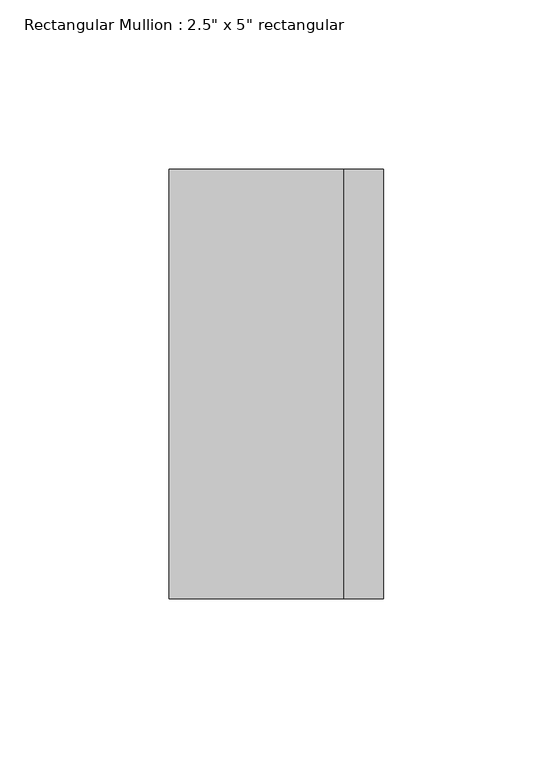
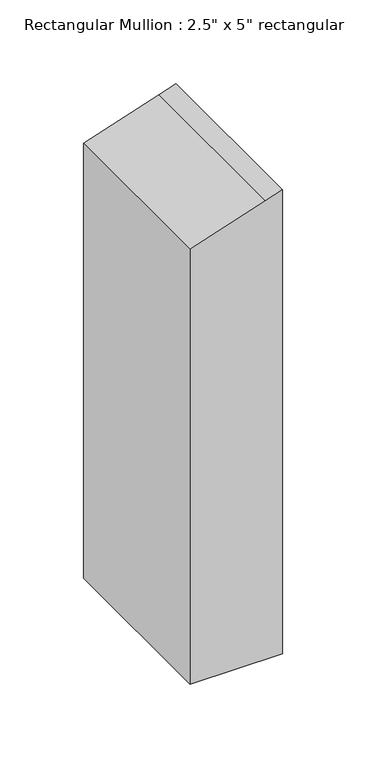
"""IFC4 building model written with IfcOpenShell, lengths in millimetres: member geometry."""

import ifcopenshell
import ifcopenshell.guid

model = None  # the IFC model being written
_history = None  # IfcOwnerHistory: only IFC2X3 demands one
_inside = {}  # id of a spatial element -> (the spatial element, [elements in it])
_under = {}  # id of a project, library or spatial element -> (it, [spatial elements below it])
_declared = {}  # id of a project -> (the project, [libraries it declares])
_typed = {}  # id of a type object -> (the type object, [elements of that type])
_made_of = {}  # id of a material, layer set ... -> (it, [elements and type objects made of it])


def new_model(schema):
    """Start an empty IFC model of exactly this schema.

    Asked for "IFC4X3", IfcOpenShell would pick the latest addendum, in which some entities
    have other attributes; the version numbers below select the first issue.
    IFC2X3 requires an IfcOwnerHistory on every rooted entity: one is made here for all.
    """
    global model, _history
    if schema == "IFC4X3":
        model = ifcopenshell.file(schema_version=(4, 3, 0, 0))
    else:
        model = ifcopenshell.file(schema=schema)
    _inside.clear()
    _under.clear()
    _declared.clear()
    _typed.clear()
    _made_of.clear()
    _history = None
    if model.schema == "IFC2X3":
        org = make("IfcOrganization", Name="unknown")
        user = make(
            "IfcPersonAndOrganization",
            ThePerson=make("IfcPerson", FamilyName="unknown"),
            TheOrganization=org,
        )
        app = make(
            "IfcApplication",
            ApplicationDeveloper=org,
            Version="unknown",
            ApplicationFullName="unknown",
            ApplicationIdentifier="unknown",
        )
        _history = make(
            "IfcOwnerHistory",
            OwningUser=user,
            OwningApplication=app,
            ChangeAction="ADDED",
            CreationDate=0,
        )
    return model


def make(cls, **values):
    """One entity of the class cls with the attributes given. An attribute that is None is left unset."""
    return model.create_entity(
        cls, **{name: value for name, value in values.items() if value is not None}
    )


def rooted(cls, **values):
    """An entity with a GlobalId (a new one), such as an element, a storey or a relation."""
    return make(cls, GlobalId=ifcopenshell.guid.new(), OwnerHistory=_history, **values)


def si_unit(unit_type, name, prefix=None):
    """IfcSIUnit, for example si_unit("LENGTHUNIT", "METRE", prefix="MILLI")."""
    return make("IfcSIUnit", UnitType=unit_type, Prefix=prefix, Name=name)


def assignment(units):
    """IfcUnitAssignment: the units of a project."""
    return None if units is None else make("IfcUnitAssignment", Units=units)


def point(xyz):
    """IfcCartesianPoint."""
    return None if xyz is None else make("IfcCartesianPoint", Coordinates=xyz)


def direction(xyz):
    """IfcDirection."""
    return None if xyz is None else make("IfcDirection", DirectionRatios=xyz)


def frame(location, z_axis=None, x_axis=None):
    """IfcAxis2Placement3D, a coordinate frame: its origin and axes. An axis left out is left unset."""
    return make(
        "IfcAxis2Placement3D",
        Location=point(location),
        Axis=direction(z_axis),
        RefDirection=direction(x_axis),
    )


def origin():
    """The frame at (0, 0, 0) with its axes left unset."""
    return frame((0.0, 0.0, 0.0))


def place(relative_to, where):
    """IfcLocalPlacement: puts the frame where relative to a parent placement (None: the world)."""
    return make(
        "IfcLocalPlacement", PlacementRelTo=relative_to, RelativePlacement=where
    )


def context(
    kind, dimensions, precision=None, world=None, true_north=None, identifier=None
):
    """IfcGeometricRepresentationContext, for example the 3D "Model" context."""
    return make(
        "IfcGeometricRepresentationContext",
        ContextIdentifier=identifier,
        ContextType=kind,
        CoordinateSpaceDimension=dimensions,
        Precision=precision,
        WorldCoordinateSystem=world,
        TrueNorth=true_north,
    )


def project(units=None, contexts=None):
    """IfcProject with its units and contexts."""
    return rooted(
        "IfcProject",
        Name="project",
        RepresentationContexts=contexts,
        UnitsInContext=assignment(units),
    )


def spatial(cls, under=None, at=None, **own):
    """A site, building, storey or space (cls), placed at a placement, below another one or the project."""
    s = rooted(cls, ObjectPlacement=at, **own)
    if under is not None:
        _under.setdefault(under.id(), (under, []))[1].append(s)
    return s


def polyline(points):
    """IfcPolyline through the points."""
    return make("IfcPolyline", Points=[point(p) for p in points])


def outline(outer, holes=None, kind="AREA"):
    """IfcArbitraryClosedProfileDef: a profile drawn as a closed curve; with holes, ...WithVoids."""
    if holes is None:
        return make("IfcArbitraryClosedProfileDef", ProfileType=kind, OuterCurve=outer)
    return make(
        "IfcArbitraryProfileDefWithVoids",
        ProfileType=kind,
        OuterCurve=outer,
        InnerCurves=holes,
    )


def extrude(swept, where, along, depth):
    """IfcExtrudedAreaSolid: the profile swept, set in the frame where, extruded along a direction by depth."""
    return make(
        "IfcExtrudedAreaSolid",
        SweptArea=swept,
        Position=where,
        ExtrudedDirection=direction(along),
        Depth=depth,
    )


def shape(context_of_items, identifier, shape_type, items):
    """IfcShapeRepresentation: the items that make up one representation, for example the "Body"."""
    return make(
        "IfcShapeRepresentation",
        ContextOfItems=context_of_items,
        RepresentationIdentifier=identifier,
        RepresentationType=shape_type,
        Items=items,
    )


def source(mapping_origin, context_of_items, identifier, shape_type, items):
    """IfcRepresentationMap: a shape defined once, which mapped items show again and again."""
    return make(
        "IfcRepresentationMap",
        MappingOrigin=mapping_origin,
        MappedRepresentation=shape(context_of_items, identifier, shape_type, items),
    )


def transform(
    local_origin,
    x_axis=None,
    y_axis=None,
    z_axis=None,
    scale=None,
    scale2=None,
    scale3=None,
    uniform=True,
):
    """IfcCartesianTransformationOperator3D, or its non-uniform kind. x_axis, y_axis, z_axis: its Axis1, 2, 3."""
    if uniform:
        return make(
            "IfcCartesianTransformationOperator3D",
            Axis1=direction(x_axis),
            Axis2=direction(y_axis),
            LocalOrigin=point(local_origin),
            Scale=scale,
            Axis3=direction(z_axis),
        )
    return make(
        "IfcCartesianTransformationOperator3DnonUniform",
        Axis1=direction(x_axis),
        Axis2=direction(y_axis),
        LocalOrigin=point(local_origin),
        Scale=scale,
        Axis3=direction(z_axis),
        Scale2=scale2,
        Scale3=scale3,
    )


def mapped(mapping_source, mapping_target):
    """IfcMappedItem: shows the shape of a source again, moved by a transform."""
    return make(
        "IfcMappedItem", MappingSource=mapping_source, MappingTarget=mapping_target
    )


def made_of(thing, what):
    """Note that an element or type object is made of a material, layer set ...; save() writes the relation."""
    if what is not None:
        _made_of.setdefault(what.id(), (what, []))[1].append(thing)
    return thing


def element(
    cls,
    number,
    at=None,
    inside=None,
    cuts=None,
    type_object=None,
    material=None,
    context=None,
    identifier="Body",
    shape_type=None,
    held_by="IfcProductDefinitionShape",
    body=None,
    shapes=None,
    **own,
):
    """One element of the class cls, such as IfcWall. Its Tag is "e" and its number.

    at: its placement. inside: the storey or other place that contains it. cuts: it is an
    opening in that element (IfcRelVoidsElement). A single representation is given by context,
    identifier, shape_type and body (its items); several are given by shapes. held_by: the class
    of the entity that holds the representations. save() writes the other relations.
    """
    e = rooted(cls, Tag="e%d" % number, ObjectPlacement=at, **own)
    if body is not None:
        shapes = [shape(context, identifier, shape_type, body)]
    if shapes is not None:
        e.Representation = make(held_by, Representations=shapes)
    if inside is not None:
        _inside.setdefault(inside.id(), (inside, []))[1].append(e)
    if cuts is not None:
        rooted(
            "IfcRelVoidsElement", RelatingBuildingElement=cuts, RelatedOpeningElement=e
        )
    if type_object is not None:
        _typed.setdefault(type_object.id(), (type_object, []))[1].append(e)
    return made_of(e, material)


def aggregate(whole, parts):
    """IfcRelAggregates: a whole, such as a stair, and the parts it consists of."""
    return rooted("IfcRelAggregates", RelatingObject=whole, RelatedObjects=parts)


def save(model, path):
    """Write the relations noted so far, then the file.

    IfcRelAggregates (storeys below a building ...), IfcRelContainedInSpatialStructure (elements
    in a storey), IfcRelDefinesByType, IfcRelAssociatesMaterial and IfcRelDeclares: one each for
    every whole, place, type object, material and project.
    """
    for whole, parts in _under.values():
        aggregate(whole, parts)
    for where, things in _inside.values():
        rooted(
            "IfcRelContainedInSpatialStructure",
            RelatedElements=things,
            RelatingStructure=where,
        )
    for kind, things in _typed.values():
        rooted("IfcRelDefinesByType", RelatedObjects=things, RelatingType=kind)
    for what, things in _made_of.values():
        rooted("IfcRelAssociatesMaterial", RelatedObjects=things, RelatingMaterial=what)
    for by, libraries in _declared.values():
        rooted("IfcRelDeclares", RelatingContext=by, RelatedDefinitions=libraries)
    model.write(path)


def member_4c11d242(model_context):
    return source(origin(), model_context, "Body", "SweptSolid", [
        extrude(outline(polyline([(-56.3515438, 31.75), (-60.2413894, 20.0804631), (-77.5182105, -31.75), (-394.1459231, -31.75), (-394.1459231, 31.75), (-56.3515438, 31.75)])), frame((0.0, -63.5, 0.0), z_axis=(0.0, 1.0, 0.0), x_axis=(0.0, 0.0, 1.0)), (0.0, 0.0, 1.0), 127.0),
    ])


if __name__ == "__main__":
    model = new_model("IFC4")
    model_context = context("Model", 3, world=origin())
    ifc_project = project(units=[si_unit("LENGTHUNIT", "METRE", prefix="MILLI")], contexts=[model_context])
    site = spatial("IfcSite", under=ifc_project)
    building = spatial("IfcBuilding", under=site)
    placement = place(None, origin())
    member_shape = member_4c11d242(model_context)
    element("IfcMember", 1, ObjectType="Rectangular Mullion : 2.5\" x 5\" rectangular", at=placement, inside=building, context=model_context, shape_type="MappedRepresentation", body=[
        mapped(member_shape, transform((0.0, 0.0, 0.0), x_axis=(1.0, 0.0, 0.0), y_axis=(0.0, 1.0, 0.0), z_axis=(0.0, 0.0, 1.0))),
    ])
    save(model, "model.ifc")

# Revit data of these elements
# Type "Rectangular Mullion : 2.5\" x 5\" rectangular"
#   built-in parameter 1007304 = 0.416667 (stored number, unit not read)
#   built-in parameter 1007301 = 0.104167 (stored number, unit not read)
#   built-in parameter 1007300 = 0.104167 (stored number, unit not read)
# Element 1 (IfcMember, "Rectangular Mullion : 2.5\" x 5\" rectangular")
#   Materials on its faces: "Metal - Aluminum, Black-Annodized"
# Materials
#   "Metal - Aluminum, Black-Annodized": class "Metal", colour RGB 10 10 10, transparency 0, Cost = 0
